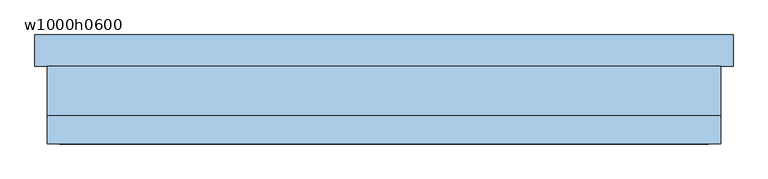
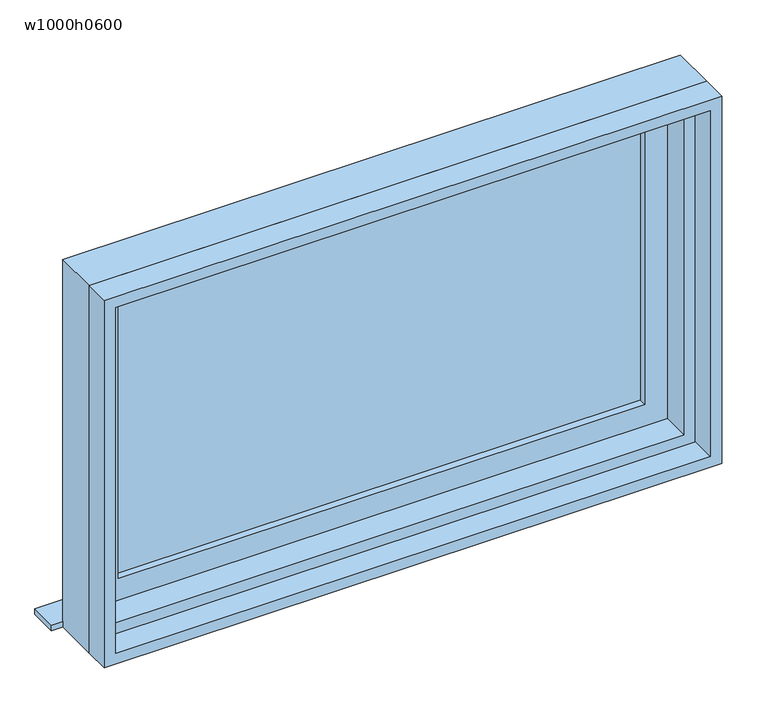
"""IFC4 building model written with IfcOpenShell, lengths in millimetres: window geometry, 横すべり窓 : w1000h0600."""

from ifc_helpers import new_model, si_unit, frame, origin, place, context, project, spatial, polyline, outline, extrude, source, transform, mapped, element, save


def w1000h0600_16d3eb2e(model_context):
    return source(origin(), model_context, "Body", "SweptSolid", [
        extrude(outline(polyline([(460.0, 22.5), (-460.0, 22.5), (-460.0, 27.5), (460.0, 27.5), (460.0, 22.5)])), frame((0.0, 0.0, 1440.0), z_axis=(0.0, 0.0, 1.0), x_axis=(1.0, 0.0, 0.0)), (0.0, 0.0, 1.0), 520.0),
        extrude(outline(polyline([(2000.0, 500.0), (2000.0, -500.0), (1400.0, -500.0), (1400.0, 500.0), (2000.0, 500.0)]), holes=[polyline([(1960.0, -460.0), (1960.0, 460.0), (1440.0, 460.0), (1440.0, -460.0), (1960.0, -460.0)])]), frame((0.0, 10.0, 0.0), z_axis=(0.0, 1.0, 0.0), x_axis=(0.0, 0.0, 1.0)), (0.0, 0.0, 1.0), 30.0),
        extrude(outline(polyline([(560.0, 90.0), (560.0, 40.0), (-560.0, 40.0), (-560.0, 90.0), (560.0, 90.0)])), frame((0.0, 0.0, 1360.0), z_axis=(0.0, 0.0, 1.0), x_axis=(1.0, 0.0, 0.0)), (0.0, 0.0, 1.0), 10.0),
        extrude(outline(polyline([(2040.0, 540.0), (2040.0, -540.0), (1360.0, -540.0), (1360.0, 540.0), (2040.0, 540.0)]), holes=[polyline([(1380.0, -520.0), (2020.0, -520.0), (2020.0, 520.0), (1380.0, 520.0), (1380.0, -520.0)])]), frame((0.0, -85.0, 0.0), z_axis=(0.0, 1.0, 0.0), x_axis=(0.0, 0.0, 1.0)), (0.0, 0.0, 1.0), 45.0),
        extrude(outline(polyline([(2040.0, -540.0), (1360.0, -540.0), (1360.0, 540.0), (2040.0, 540.0), (2040.0, -540.0)]), holes=[polyline([(2000.0, 500.0), (1400.0, 500.0), (1400.0, -500.0), (2000.0, -500.0), (2000.0, 500.0)])]), frame((0.0, -40.0, 0.0), z_axis=(0.0, 1.0, 0.0), x_axis=(0.0, 0.0, 1.0)), (0.0, 0.0, 1.0), 80.0),
    ])


if __name__ == "__main__":
    model = new_model("IFC4")
    model_context = context("Model", 3, world=origin())
    ifc_project = project(units=[si_unit("LENGTHUNIT", "METRE", prefix="MILLI")], contexts=[model_context])
    site = spatial("IfcSite", under=ifc_project)
    building = spatial("IfcBuilding", under=site)
    placement = place(None, origin())
    w1000h0600_shape = w1000h0600_16d3eb2e(model_context)
    element("IfcWindow", 1, ObjectType="横すべり窓 : w1000h0600", at=placement, inside=building, context=model_context, shape_type="MappedRepresentation", body=[
        mapped(w1000h0600_shape, transform((0.0, 0.0, 0.0), x_axis=(1.0, 0.0, 0.0), y_axis=(0.0, 1.0, 0.0), z_axis=(0.0, 0.0, 1.0))),
    ])
    save(model, "model.ifc")

# Revit data of these elements
# Type "横すべり窓 : w1000h0600"
#   Construction Type Id = "GSP4R"
#   Analytic Construction = "1/8 インチ ピルキントン一重ガラス"
#   Type Mark = "78"
#   Operation = "シングルパネル"
#   Keynote = "08520.S1"
#   Visual Light Transmittance = 0.9
#   Solar Heat Gain Coefficient = 0.86
#   Heat Transfer Coefficient (U) = 6.7069 W/(m²·K)
#   Height = 600 mm
#   既定の腰高 = 1400 mm
#   Width = 1000 mm
#   額縁見附 = 20 mm
#   額縁ちり = 10 mm
#   サッシ見附 = 40 mm
#   サッシの幅 = 80 mm
#   サッシ額縁 [instance default] = none
#   サッシ本体 [instance default] = none
#   サッシガラス [instance default] = ガラス - 透明
#   Wall Closure = (empty or 0)
#   Type Comments = ""
#   Assembly Code = ""
# Element 1 (IfcWindow, "横すべり窓 : w1000h0600")
#   Materials on its faces: "ガラス - 透明"
# Materials
#   "ガラス - 透明": class "ガラス", colour RGB 0 128 192, transparency 0.9, Cost = 0
